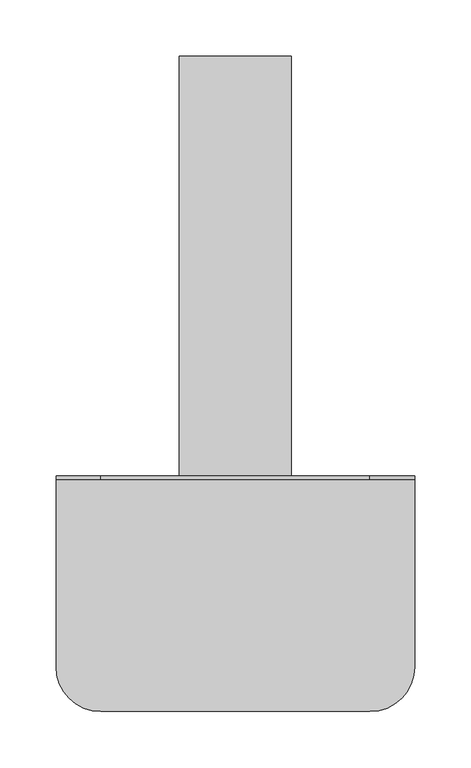
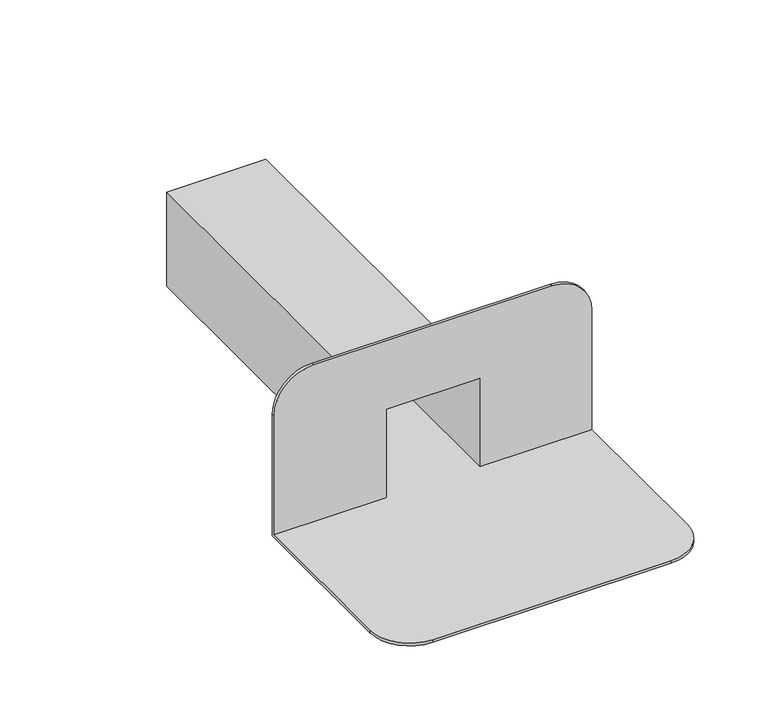
"""IFC4 building model written with IfcOpenShell, lengths in millimetres: proxy geometry, TN_ПВХ воронка парапетная : ПВХ воронка парапетная 100х100мм длиной 375мм."""

import ifcopenshell
import ifcopenshell.guid

model = None  # the IFC model being written
_history = None  # IfcOwnerHistory: only IFC2X3 demands one
_inside = {}  # id of a spatial element -> (the spatial element, [elements in it])
_under = {}  # id of a project, library or spatial element -> (it, [spatial elements below it])
_declared = {}  # id of a project -> (the project, [libraries it declares])
_typed = {}  # id of a type object -> (the type object, [elements of that type])
_made_of = {}  # id of a material, layer set ... -> (it, [elements and type objects made of it])


def new_model(schema):
    """Start an empty IFC model of exactly this schema.

    Asked for "IFC4X3", IfcOpenShell would pick the latest addendum, in which some entities
    have other attributes; the version numbers below select the first issue.
    IFC2X3 requires an IfcOwnerHistory on every rooted entity: one is made here for all.
    """
    global model, _history
    if schema == "IFC4X3":
        model = ifcopenshell.file(schema_version=(4, 3, 0, 0))
    else:
        model = ifcopenshell.file(schema=schema)
    _inside.clear()
    _under.clear()
    _declared.clear()
    _typed.clear()
    _made_of.clear()
    _history = None
    if model.schema == "IFC2X3":
        org = make("IfcOrganization", Name="unknown")
        user = make(
            "IfcPersonAndOrganization",
            ThePerson=make("IfcPerson", FamilyName="unknown"),
            TheOrganization=org,
        )
        app = make(
            "IfcApplication",
            ApplicationDeveloper=org,
            Version="unknown",
            ApplicationFullName="unknown",
            ApplicationIdentifier="unknown",
        )
        _history = make(
            "IfcOwnerHistory",
            OwningUser=user,
            OwningApplication=app,
            ChangeAction="ADDED",
            CreationDate=0,
        )
    return model


def make(cls, **values):
    """One entity of the class cls with the attributes given. An attribute that is None is left unset."""
    return model.create_entity(
        cls, **{name: value for name, value in values.items() if value is not None}
    )


def rooted(cls, **values):
    """An entity with a GlobalId (a new one), such as an element, a storey or a relation."""
    return make(cls, GlobalId=ifcopenshell.guid.new(), OwnerHistory=_history, **values)


def si_unit(unit_type, name, prefix=None):
    """IfcSIUnit, for example si_unit("LENGTHUNIT", "METRE", prefix="MILLI")."""
    return make("IfcSIUnit", UnitType=unit_type, Prefix=prefix, Name=name)


def assignment(units):
    """IfcUnitAssignment: the units of a project."""
    return None if units is None else make("IfcUnitAssignment", Units=units)


def point(xyz):
    """IfcCartesianPoint."""
    return None if xyz is None else make("IfcCartesianPoint", Coordinates=xyz)


def direction(xyz):
    """IfcDirection."""
    return None if xyz is None else make("IfcDirection", DirectionRatios=xyz)


def frame(location, z_axis=None, x_axis=None):
    """IfcAxis2Placement3D, a coordinate frame: its origin and axes. An axis left out is left unset."""
    return make(
        "IfcAxis2Placement3D",
        Location=point(location),
        Axis=direction(z_axis),
        RefDirection=direction(x_axis),
    )


def origin():
    """The frame at (0, 0, 0) with its axes left unset."""
    return frame((0.0, 0.0, 0.0))


def place(relative_to, where):
    """IfcLocalPlacement: puts the frame where relative to a parent placement (None: the world)."""
    return make(
        "IfcLocalPlacement", PlacementRelTo=relative_to, RelativePlacement=where
    )


def context(
    kind, dimensions, precision=None, world=None, true_north=None, identifier=None
):
    """IfcGeometricRepresentationContext, for example the 3D "Model" context."""
    return make(
        "IfcGeometricRepresentationContext",
        ContextIdentifier=identifier,
        ContextType=kind,
        CoordinateSpaceDimension=dimensions,
        Precision=precision,
        WorldCoordinateSystem=world,
        TrueNorth=true_north,
    )


def project(units=None, contexts=None):
    """IfcProject with its units and contexts."""
    return rooted(
        "IfcProject",
        Name="project",
        RepresentationContexts=contexts,
        UnitsInContext=assignment(units),
    )


def spatial(cls, under=None, at=None, **own):
    """A site, building, storey or space (cls), placed at a placement, below another one or the project."""
    s = rooted(cls, ObjectPlacement=at, **own)
    if under is not None:
        _under.setdefault(under.id(), (under, []))[1].append(s)
    return s


def circle_curve(where, radius):
    """IfcCircle in the frame where."""
    return make("IfcCircle", Position=where, Radius=radius)


def shape(context_of_items, identifier, shape_type, items):
    """IfcShapeRepresentation: the items that make up one representation, for example the "Body"."""
    return make(
        "IfcShapeRepresentation",
        ContextOfItems=context_of_items,
        RepresentationIdentifier=identifier,
        RepresentationType=shape_type,
        Items=items,
    )


def source(mapping_origin, context_of_items, identifier, shape_type, items):
    """IfcRepresentationMap: a shape defined once, which mapped items show again and again."""
    return make(
        "IfcRepresentationMap",
        MappingOrigin=mapping_origin,
        MappedRepresentation=shape(context_of_items, identifier, shape_type, items),
    )


def transform(
    local_origin,
    x_axis=None,
    y_axis=None,
    z_axis=None,
    scale=None,
    scale2=None,
    scale3=None,
    uniform=True,
):
    """IfcCartesianTransformationOperator3D, or its non-uniform kind. x_axis, y_axis, z_axis: its Axis1, 2, 3."""
    if uniform:
        return make(
            "IfcCartesianTransformationOperator3D",
            Axis1=direction(x_axis),
            Axis2=direction(y_axis),
            LocalOrigin=point(local_origin),
            Scale=scale,
            Axis3=direction(z_axis),
        )
    return make(
        "IfcCartesianTransformationOperator3DnonUniform",
        Axis1=direction(x_axis),
        Axis2=direction(y_axis),
        LocalOrigin=point(local_origin),
        Scale=scale,
        Axis3=direction(z_axis),
        Scale2=scale2,
        Scale3=scale3,
    )


def mapped(mapping_source, mapping_target):
    """IfcMappedItem: shows the shape of a source again, moved by a transform."""
    return make(
        "IfcMappedItem", MappingSource=mapping_source, MappingTarget=mapping_target
    )


def made_of(thing, what):
    """Note that an element or type object is made of a material, layer set ...; save() writes the relation."""
    if what is not None:
        _made_of.setdefault(what.id(), (what, []))[1].append(thing)
    return thing


def element(
    cls,
    number,
    at=None,
    inside=None,
    cuts=None,
    type_object=None,
    material=None,
    context=None,
    identifier="Body",
    shape_type=None,
    held_by="IfcProductDefinitionShape",
    body=None,
    shapes=None,
    **own,
):
    """One element of the class cls, such as IfcWall. Its Tag is "e" and its number.

    at: its placement. inside: the storey or other place that contains it. cuts: it is an
    opening in that element (IfcRelVoidsElement). A single representation is given by context,
    identifier, shape_type and body (its items); several are given by shapes. held_by: the class
    of the entity that holds the representations. save() writes the other relations.
    """
    e = rooted(cls, Tag="e%d" % number, ObjectPlacement=at, **own)
    if body is not None:
        shapes = [shape(context, identifier, shape_type, body)]
    if shapes is not None:
        e.Representation = make(held_by, Representations=shapes)
    if inside is not None:
        _inside.setdefault(inside.id(), (inside, []))[1].append(e)
    if cuts is not None:
        rooted(
            "IfcRelVoidsElement", RelatingBuildingElement=cuts, RelatedOpeningElement=e
        )
    if type_object is not None:
        _typed.setdefault(type_object.id(), (type_object, []))[1].append(e)
    return made_of(e, material)


def aggregate(whole, parts):
    """IfcRelAggregates: a whole, such as a stair, and the parts it consists of."""
    return rooted("IfcRelAggregates", RelatingObject=whole, RelatedObjects=parts)


def save(model, path):
    """Write the relations noted so far, then the file.

    IfcRelAggregates (storeys below a building ...), IfcRelContainedInSpatialStructure (elements
    in a storey), IfcRelDefinesByType, IfcRelAssociatesMaterial and IfcRelDeclares: one each for
    every whole, place, type object, material and project.
    """
    for whole, parts in _under.values():
        aggregate(whole, parts)
    for where, things in _inside.values():
        rooted(
            "IfcRelContainedInSpatialStructure",
            RelatedElements=things,
            RelatingStructure=where,
        )
    for kind, things in _typed.values():
        rooted("IfcRelDefinesByType", RelatedObjects=things, RelatingType=kind)
    for what, things in _made_of.values():
        rooted("IfcRelAssociatesMaterial", RelatedObjects=things, RelatingMaterial=what)
    for by, libraries in _declared.values():
        rooted("IfcRelDeclares", RelatingContext=by, RelatedDefinitions=libraries)
    model.write(path)


def plane_surface(at):
    """IfcPlane: the flat surface through the origin of the frame at, square to its z axis."""
    return make("IfcPlane", Position=at)


def cylinder_surface(at, radius):
    """IfcCylindricalSurface: all points at the distance radius from the z axis of the frame at."""
    return make("IfcCylindricalSurface", Position=at, Radius=radius)


def advanced_brep(points, edges, surfaces, faces):
    """IfcAdvancedBrep: a solid bounded by faces that lie on surfaces and meet in shared edges.

    An edge is (start, end): straight between two places in points (the first is 0);
    or (start, end, curve); or (start, end, curve, False) where it runs against its curve.
    A face is (place in surfaces, loops), or (place, loops, False) where it looks against
    its surface's normal. A loop lists edges by number (the first is 1), with a minus sign
    where the edge is run from its end to its start. The first loop is the outer one.
    """
    corners = [point(p) for p in points]
    vertices = [make("IfcVertexPoint", VertexGeometry=c) for c in corners]
    made = []
    for start, end, *more in edges:
        made.append(
            make(
                "IfcEdgeCurve",
                EdgeStart=vertices[start],
                EdgeEnd=vertices[end],
                EdgeGeometry=more[0] if more else make("IfcPolyline", Points=[corners[start], corners[end]]),
                SameSense=more[1] if len(more) > 1 else True,
            )
        )
    hull = []
    for where, loops, *sense in faces:
        bounds = []
        for j, loop in enumerate(loops):
            ring = [make("IfcOrientedEdge", EdgeElement=made[abs(k) - 1], Orientation=k > 0) for k in loop]
            bounds.append(
                make(
                    "IfcFaceOuterBound" if j == 0 else "IfcFaceBound",
                    Bound=make("IfcEdgeLoop", EdgeList=ring),
                    Orientation=True,
                )
            )
        hull.append(make("IfcAdvancedFace", Bounds=bounds, FaceSurface=surfaces[where], SameSense=sense[0] if sense else True))
    return make("IfcAdvancedBrep", Outer=make("IfcClosedShell", CfsFaces=hull))


def specialty_equipment_2792bfd9(model_context):
    return source(origin(), model_context, "Body", "AdvancedBrep", [
        advanced_brep(
        [(50.0, 375.0, 0.0), (-50.0, 375.0, 0.0), (-50.0, 375.0, 100.0), (50.0, 375.0, 100.0), (47.0, 375.0, 3.0), (47.0, 375.0, 97.0), (-47.0, 375.0, 97.0), (-47.0, 375.0, 3.0), (50.0, 0.0, 100.0), (50.0, 0.0, 0.0), (-50.0, 0.0, 100.0), (-50.0, 0.0, 0.0), (160.0, 0.0, 0.0), (160.0, -170.0, 0.0), (120.0, -210.0, 0.0), (-120.0, -210.0, 0.0), (-160.0, -170.0, 0.0), (-160.0, 0.0, 0.0), (-47.0, -3.0, 3.0), (-160.0, -3.0, 3.0), (-160.0, -170.0, 3.0), (-120.0, -210.0, 3.0), (120.0, -210.0, 3.0), (160.0, -170.0, 3.0), (160.0, -3.0, 3.0), (47.0, -3.0, 3.0), (-47.0, -3.0, 97.0), (47.0, -3.0, 97.0), (160.0, -3.0, 130.0), (120.0, -3.0, 170.0), (-120.0, -3.0, 170.0), (-160.0, -3.0, 130.0), (-160.0, 0.0, 130.0), (-120.0, 0.0, 170.0), (120.0, 0.0, 170.0), (160.0, 0.0, 130.0)],
        [
            (0, 1),
            (1, 2),
            (2, 3),
            (3, 0),
            (4, 5),
            (5, 6),
            (6, 7),
            (7, 4),
            (3, 8),
            (8, 9),
            (9, 0),
            (2, 10),
            (10, 8),
            (1, 11),
            (11, 10),
            (9, 12),
            (12, 13),
            (13, 14, circle_curve(frame((120.0, -170.0, 0.0), z_axis=(0.0, 0.0, -1.0), x_axis=(1.0, 0.0, 0.0)), 40.0)),
            (14, 15),
            (15, 16, circle_curve(frame((-120.0, -170.0, 0.0), z_axis=(0.0, 0.0, -1.0), x_axis=(1.0, 0.0, 0.0)), 40.0)),
            (16, 17),
            (17, 11),
            (7, 18),
            (18, 19),
            (19, 20),
            (20, 21, circle_curve(frame((-120.0, -170.0, 3.0), z_axis=(0.0, 0.0, 1.0), x_axis=(1.0, 0.0, 0.0)), 40.0)),
            (21, 22),
            (22, 23, circle_curve(frame((120.0, -170.0, 3.0), z_axis=(0.0, 0.0, 1.0), x_axis=(1.0, 0.0, 0.0)), 40.0)),
            (23, 24),
            (24, 25),
            (25, 4),
            (6, 26),
            (26, 18),
            (5, 27),
            (27, 26),
            (25, 27),
            (24, 28),
            (28, 29, circle_curve(frame((120.0, -3.0, 130.0), z_axis=(0.0, -1.0, 0.0), x_axis=(1.0, 0.0, 0.0)), 40.0)),
            (29, 30),
            (30, 31, circle_curve(frame((-120.0, -3.0, 130.0), z_axis=(0.0, -1.0, 0.0), x_axis=(1.0, 0.0, 0.0)), 40.0)),
            (31, 19),
            (32, 33, circle_curve(frame((-120.0, 0.0, 130.0), z_axis=(0.0, 1.0, 0.0), x_axis=(1.0, 0.0, 0.0)), 40.0)),
            (33, 34),
            (34, 35, circle_curve(frame((120.0, 0.0, 130.0), z_axis=(0.0, 1.0, 0.0), x_axis=(1.0, 0.0, 0.0)), 40.0)),
            (35, 12),
            (17, 32),
            (23, 13),
            (35, 28),
            (34, 29),
            (33, 30),
            (32, 31),
            (16, 20),
            (15, 21),
            (14, 22),
        ],
        [
            plane_surface(frame((50.0, 375.0, 0.0), z_axis=(0.0, 1.0, 0.0), x_axis=(0.0, 0.0, -1.0))),
            plane_surface(frame((50.0, 0.0, 0.0), z_axis=(1.0, 0.0, 0.0), x_axis=(0.0, 1.0, 0.0))),
            plane_surface(frame((50.0, 0.0, 100.0), z_axis=(0.0, 0.0, 1.0), x_axis=(0.0, 1.0, 0.0))),
            plane_surface(frame((-50.0, 0.0, 100.0), z_axis=(-1.0, 0.0, 0.0), x_axis=(0.0, 1.0, 0.0))),
            plane_surface(frame((-50.0, 0.0, 0.0), z_axis=(0.0, 0.0, -1.0), x_axis=(0.0, 1.0, 0.0))),
            plane_surface(frame((47.0, 0.0, 3.0), z_axis=(0.0, 0.0, 1.0), x_axis=(0.0, 1.0, 0.0))),
            plane_surface(frame((-47.0, 0.0, 3.0), z_axis=(1.0, 0.0, 0.0), x_axis=(0.0, 1.0, 0.0))),
            plane_surface(frame((-47.0, 0.0, 97.0), z_axis=(0.0, 0.0, -1.0), x_axis=(0.0, 1.0, 0.0))),
            plane_surface(frame((47.0, 0.0, 97.0), z_axis=(-1.0, 0.0, 0.0), x_axis=(0.0, 1.0, 0.0))),
            plane_surface(frame((160.0, -3.0, 130.0), z_axis=(0.0, -1.0, 0.0), x_axis=(0.0, 0.0, 1.0))),
            plane_surface(frame((160.0, 0.0, 130.0), z_axis=(0.0, 1.0, 0.0), x_axis=(0.0, 0.0, -1.0))),
            plane_surface(frame((160.0, -3.0, 3.0), z_axis=(1.0, 0.0, 0.0), x_axis=(0.0, 1.0, 0.0))),
            cylinder_surface(frame((120.0, 0.0, 130.0), z_axis=(0.0, -1.0, 0.0), x_axis=(1.0, 0.0, 0.0)), 40.0),
            plane_surface(frame((120.0, -3.0, 170.0), z_axis=(0.0, 0.0, 1.0), x_axis=(0.0, 1.0, 0.0))),
            cylinder_surface(frame((-120.0, 0.0, 130.0), z_axis=(0.0, -1.0, 0.0), x_axis=(1.0, 0.0, 0.0)), 40.0),
            plane_surface(frame((-160.0, -3.0, 130.0), z_axis=(-1.0, 0.0, 0.0), x_axis=(0.0, 1.0, 0.0))),
            cylinder_surface(frame((-120.0, -170.0, 0.0), z_axis=(0.0, 0.0, 1.0), x_axis=(1.0, 0.0, 0.0)), 40.0),
            plane_surface(frame((-120.0, -210.0, 3.0), z_axis=(0.0, -1.0, 0.0), x_axis=(0.0, 0.0, -1.0))),
            cylinder_surface(frame((120.0, -170.0, 0.0), z_axis=(0.0, 0.0, 1.0), x_axis=(1.0, 0.0, 0.0)), 40.0),
        ],
        [
            (0, [[1, 2, 3, 4], [5, 6, 7, 8]]),
            (1, [[-4, 9, 10, 11]]),
            (2, [[-3, 12, 13, -9]]),
            (3, [[-2, 14, 15, -12]]),
            (4, [[-1, -11, 16, 17, 18, 19, 20, 21, 22, -14]]),
            (5, [[-8, 23, 24, 25, 26, 27, 28, 29, 30, 31]]),
            (6, [[-23, -7, 32, 33]]),
            (7, [[-6, 34, 35, -32]]),
            (8, [[-5, -31, 36, -34]]),
            (9, [[37, 38, 39, 40, 41, -24, -33, -35, -36, -30]]),
            (10, [[42, 43, 44, 45, -16, -10, -13, -15, -22, 46]]),
            (11, [[-37, -29, 47, -17, -45, 48]]),
            (12, [[-38, -48, -44, 49]]),
            (13, [[-39, -49, -43, 50]]),
            (14, [[-40, -50, -42, 51]]),
            (15, [[-41, -51, -46, -21, 52, -25]]),
            (16, [[-26, -52, -20, 53]]),
            (17, [[-27, -53, -19, 54]]),
            (18, [[-28, -54, -18, -47]]),
        ],
    ),
    ])


if __name__ == "__main__":
    model = new_model("IFC4")
    model_context = context("Model", 3, world=origin())
    ifc_project = project(units=[si_unit("LENGTHUNIT", "METRE", prefix="MILLI")], contexts=[model_context])
    site = spatial("IfcSite", under=ifc_project)
    building = spatial("IfcBuilding", under=site)
    placement = place(None, origin())
    specialty_equipment_shape = specialty_equipment_2792bfd9(model_context)
    element("IfcBuildingElementProxy", 1, Name="TN_ПВХ воронка парапетная : ПВХ воронка парапетная 100х100мм длиной 375мм", ObjectType="TN_ПВХ воронка парапетная : ПВХ воронка парапетная 100х100мм длиной 375мм", at=placement, inside=building, context=model_context, shape_type="MappedRepresentation", body=[
        mapped(specialty_equipment_shape, transform((0.0, 0.0, 0.0), x_axis=(1.0, 0.0, 0.0), y_axis=(0.0, 1.0, 0.0), z_axis=(0.0, 0.0, 1.0))),
    ])
    save(model, "model.ifc")

# Revit data of these elements
# Type "TN_ПВХ воронка парапетная : ПВХ воронка парапетная 100х100мм длиной 375мм"
#   ADSK_Группирование = "Комплектующие и воронки"
#   Description = "ПВХ воронка парапетная 100x100мм с отводом L=375 мм Парапетная воронка изготавливается из высококачественного поливинилхлорида. Используется на плоских кровлях из ПВХ мембран с внешним водостоком. Воронка имеет квадратное сечение и служит для отвода воды через парапеты, балконы."
#   Manufacturer = "ТехноНИКОЛЬ"
#   URL = "https://www.tstn.ru/product/pvkh-voronka-parapetnaya-tekhnonikol-100kh100-489847/"
#   ADSK_Примечание = ""
#   ADSK_Обозначение = "ТехноНИКОЛЬ"
#   ADSK_Наименование = "ПВХ воронка парапетная ТехноНИКОЛЬ 100х100"
#   ADSK_Марка = ""
#   ADSK_Код изделия = "489847"
#   ADSK_Завод-изготовитель = "ТехноНИКОЛЬ"
#   ADSK_Единица измерения = "шт."
#   ADSK_Группирование = "Комплектующие и воронки"
#   ADSK_URL страницы изделия = "https://www.tstn.ru/product/pvkh-voronka-parapetnaya-tekhnonikol-100kh100-489847/"
#   ADSK_URL документации изделия = ""
#   Тип воронки = 2
#   Длина расчетная [instance default] = 375 mm
#   Длина отвода [instance default] = 375 mm
#   ADSK_Размер_Ширина = 100 mm
#   ADSK_Размер_Высота = 100 mm
#   ADSK_Количество = 1
#   Видимость_Переход [instance default] = no
#   Видимость_Листоуловитель [instance default] = no
#   Видимость отвода [instance default] = no
#   Видимость листоуловителя [instance default] = no
#   Материал_Листоуловитель = TN_ПВХ_Черный
#   Материал_Корпус = TN_ПВХ_Серый
#   Default Elevation = 0
# Element 1 (IfcBuildingElementProxy, "TN_ПВХ воронка парапетная : ПВХ воронка парапетная 100х100мм длиной 375мм")
#   Materials on its faces: "TN_ПВХ_Серый"
# Materials
#   "TN_ПВХ_Черный": class "Типовые", colour RGB 48 48 48, transparency 0, Cost = 0
#   "TN_ПВХ_Серый": class "Типовые", colour RGB 192 192 192, transparency 0, Cost = 0
